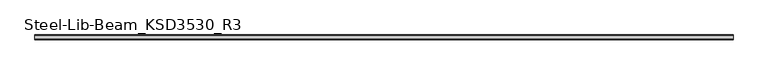
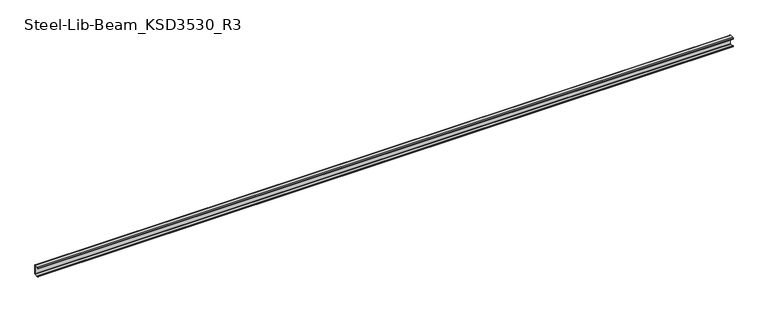
"""IFC4 building model written with IfcOpenShell, lengths in millimetres: beam geometry, Steel-Lib-Beam_KSD3530_R3 : BMS291_C-150×75x20x4.5."""

from ifc_helpers import new_model, si_unit, point, frame, frame_2d, origin, place, context, project, spatial, polyline, circle_curve, trimmed, segment, composite_curve, outline, extrude, source, transform, mapped, element, save


def steel_lib_beam_ksd3530_r3_c0f395b9(model_context):
    return source(origin(), model_context, "Body", "SweptSolid", [
        extrude(outline(composite_curve([segment(trimmed(circle_curve(frame_2d((-41.0, 66.0)), 9.0), [point((-50.0, 66.0))], [point((-41.0, 75.0))], False, "CARTESIAN"), True, "CONTINUOUS"), segment(polyline([(-41.0, 75.0), (16.0, 75.0)]), True, "CONTINUOUS"), segment(trimmed(circle_curve(frame_2d((16.0, 66.0)), 9.0), [point((16.0, 75.0))], [point((25.0, 66.0))], False, "CARTESIAN"), True, "CONTINUOUS"), segment(polyline([(25.0, 66.0), (25.0, -66.0)]), True, "CONTINUOUS"), segment(trimmed(circle_curve(frame_2d((16.0, -66.0)), 9.0), [point((25.0, -66.0))], [point((16.0, -75.0))], False, "CARTESIAN"), True, "CONTINUOUS"), segment(polyline([(16.0, -75.0), (-41.0, -75.0)]), True, "CONTINUOUS"), segment(trimmed(circle_curve(frame_2d((-41.0, -66.0)), 9.0), [point((-41.0, -75.0))], [point((-50.0, -66.0))], False, "CARTESIAN"), True, "CONTINUOUS"), segment(polyline([(-50.0, -66.0), (-50.0, -55.0), (-45.5, -55.0), (-45.5, -66.0)]), True, "CONTINUOUS"), segment(trimmed(circle_curve(frame_2d((-41.0, -66.0)), 4.5), [point((-45.5, -66.0))], [point((-41.0, -70.5))], True, "CARTESIAN"), True, "CONTINUOUS"), segment(polyline([(-41.0, -70.5), (16.0, -70.5)]), True, "CONTINUOUS"), segment(trimmed(circle_curve(frame_2d((16.0, -66.0)), 4.5), [point((16.0, -70.5))], [point((20.5, -66.0))], True, "CARTESIAN"), True, "CONTINUOUS"), segment(polyline([(20.5, -66.0), (20.5, 66.0)]), True, "CONTINUOUS"), segment(trimmed(circle_curve(frame_2d((16.0, 66.0)), 4.5), [point((20.5, 66.0))], [point((16.0, 70.5))], True, "CARTESIAN"), True, "CONTINUOUS"), segment(polyline([(16.0, 70.5), (-41.0, 70.5)]), True, "CONTINUOUS"), segment(trimmed(circle_curve(frame_2d((-41.0, 66.0)), 4.5), [point((-41.0, 70.5))], [point((-45.5, 66.0))], True, "CARTESIAN"), True, "CONTINUOUS"), segment(polyline([(-45.5, 66.0), (-45.5, 55.0), (-50.0, 55.0), (-50.0, 66.0)]), True, "CONTINUOUS")], self_intersect=False)), frame((-5215.0, 0.0, 0.0), z_axis=(1.0, 0.0, 0.0), x_axis=(0.0, 1.0, 0.0)), (0.0, 0.0, 1.0), 10430.0),
    ])


if __name__ == "__main__":
    model = new_model("IFC4")
    model_context = context("Model", 3, world=origin())
    ifc_project = project(units=[si_unit("LENGTHUNIT", "METRE", prefix="MILLI")], contexts=[model_context])
    site = spatial("IfcSite", under=ifc_project)
    building = spatial("IfcBuilding", under=site)
    placement = place(None, origin())
    steel_lib_beam_ksd3530_r3_shape = steel_lib_beam_ksd3530_r3_c0f395b9(model_context)
    element("IfcBeam", 1, ObjectType="Steel-Lib-Beam_KSD3530_R3 : BMS291_C-150×75x20x4.5", at=placement, inside=building, context=model_context, shape_type="MappedRepresentation", body=[
        mapped(steel_lib_beam_ksd3530_r3_shape, transform((0.0, 0.0, 0.0), x_axis=(1.0, 0.0, 0.0), y_axis=(0.0, 1.0, 0.0), z_axis=(0.0, 0.0, 1.0))),
    ])
    save(model, "model.ifc")

# Revit data of these elements
# Type "Steel-Lib-Beam_KSD3530_R3 : BMS291_C-150×75x20x4.5"
#   Keynote = "C-150×75x20x4.5"
#   SteelWeight = "Light"
#   x = 0.0250 m
#   t1 = 0.0090 m
#   t = 0.0045 m
#   Surface Area = 0.629834 m²/m
#   Section Area = 13.9688 cm²
#   Mass per Unit Length = 10.9655 kg/m
#   C = 0.0200 m
#   A = 0.0750 m
#   Length [instance default] = 1.5000 m
#   H = 0.1500 m
#   hec_material4 [instance default] = none
#   hec_material3 [instance default] = none
#   hec_material2 [instance default] = none
#   hec_material1 [instance default] = none
#   Structural Material [instance default] = Metal - Steel - Light Gauge
#   Assembly Code = ""
# Element 1 (IfcBeam, "Steel-Lib-Beam_KSD3530_R3 : BMS291_C-150×75x20x4.5")
#   Structural Material = none
# Materials
#   "Metal - Steel - Light Gauge": class "Metal", colour RGB 247 247 247, transparency 0
